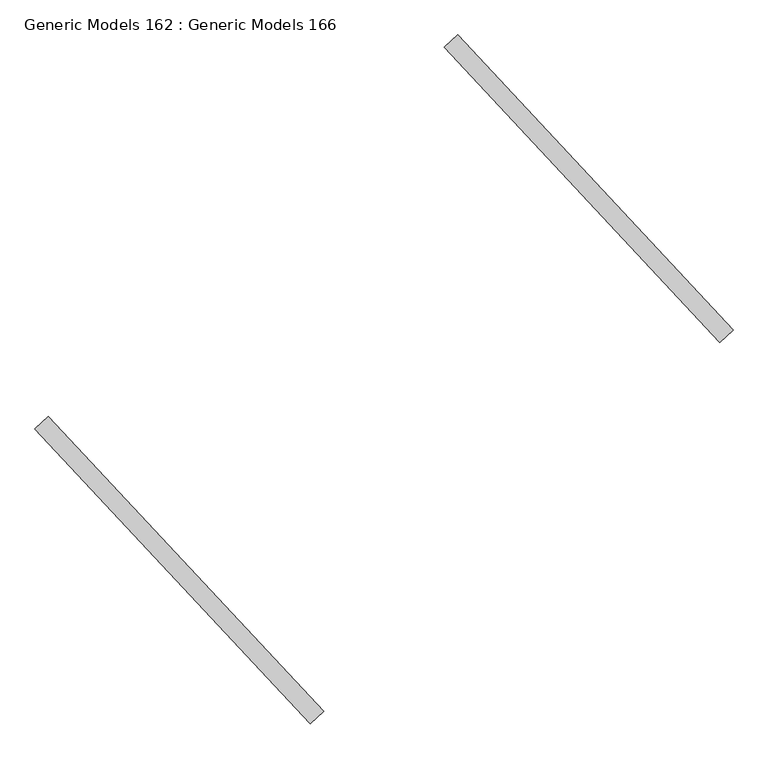
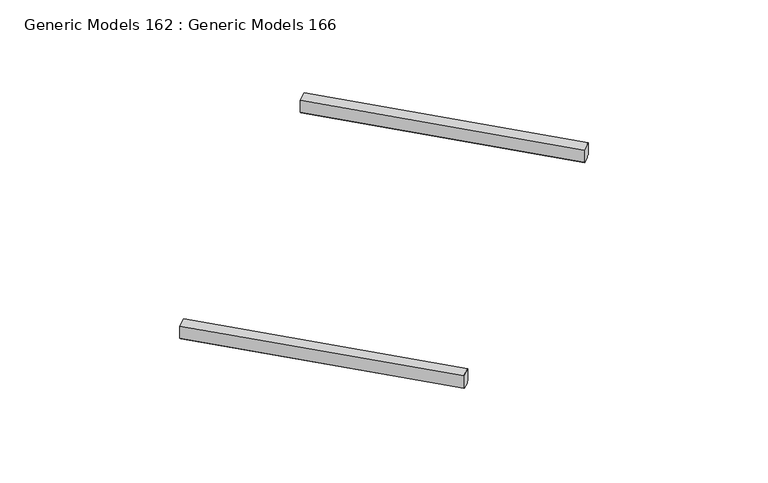
"""IFC4 building model written with IfcOpenShell, lengths in millimetres: proxy geometry, Generic Models 162 : Generic Models 166."""

from ifc_helpers import new_model, si_unit, frame, origin, place, context, project, spatial, polyline, outline, extrude, source, transform, mapped, element, save


def generic_models_162_generic_models_166_5ced6224(model_context):
    return source(origin(), model_context, "Body", "SweptSolid", [
        extrude(outline(polyline([(156.765625, -63.5000001), (17.065625, -63.5000001), (17.065625, -44.45), (0.0, -44.45), (0.0, 44.45), (17.065625, 44.45), (17.065625, 63.5), (156.765625, 63.5), (156.765625, -63.5000001)])), frame((7709.1694874, -21396.392229, 2082.8), z_axis=(-0.6819983600624979, 0.731353701619171, 0.0), x_axis=(0.0, 0.0, 1.0)), (0.0, 0.0, 1.0), 2800.35),
        extrude(outline(polyline([(156.765625, -63.4999999), (17.065625, -63.4999999), (17.065625, -44.45), (0.0, -44.45), (0.0, 44.45), (17.065625, 44.45), (17.065625, 63.5000001), (156.765625, 63.5000001), (156.765625, -63.4999999)])), frame((4866.9827321, -24046.7742559, 2082.8), z_axis=(-0.6819983600624979, 0.731353701619171, 0.0), x_axis=(0.0, 0.0, 1.0)), (0.0, 0.0, 1.0), 2800.35),
    ])


if __name__ == "__main__":
    model = new_model("IFC4")
    model_context = context("Model", 3, world=origin())
    ifc_project = project(units=[si_unit("LENGTHUNIT", "METRE", prefix="MILLI")], contexts=[model_context])
    site = spatial("IfcSite", under=ifc_project)
    building = spatial("IfcBuilding", under=site)
    placement = place(None, origin())
    generic_models_162_generic_models_166_shape = generic_models_162_generic_models_166_5ced6224(model_context)
    element("IfcBuildingElementProxy", 1, Name="Generic Models 162 : Generic Models 166", ObjectType="Generic Models 162 : Generic Models 166", at=placement, inside=building, context=model_context, shape_type="MappedRepresentation", body=[
        mapped(generic_models_162_generic_models_166_shape, transform((0.0, 0.0, 0.0), x_axis=(1.0, 0.0, 0.0), y_axis=(0.0, 1.0, 0.0), z_axis=(0.0, 0.0, 1.0))),
    ])
    save(model, "model.ifc")

# Revit data of these elements
# Element 1 (IfcBuildingElementProxy, "Generic Models 162 : Generic Models 166")
#   Materials on its faces: "2 x 4 WOOD STUDS"
# Materials
#   "2 x 4 WOOD STUDS": class "Wood", colour RGB 144 113 62, transparency 0, Description = "Pinus Echinata", Cost = 0
